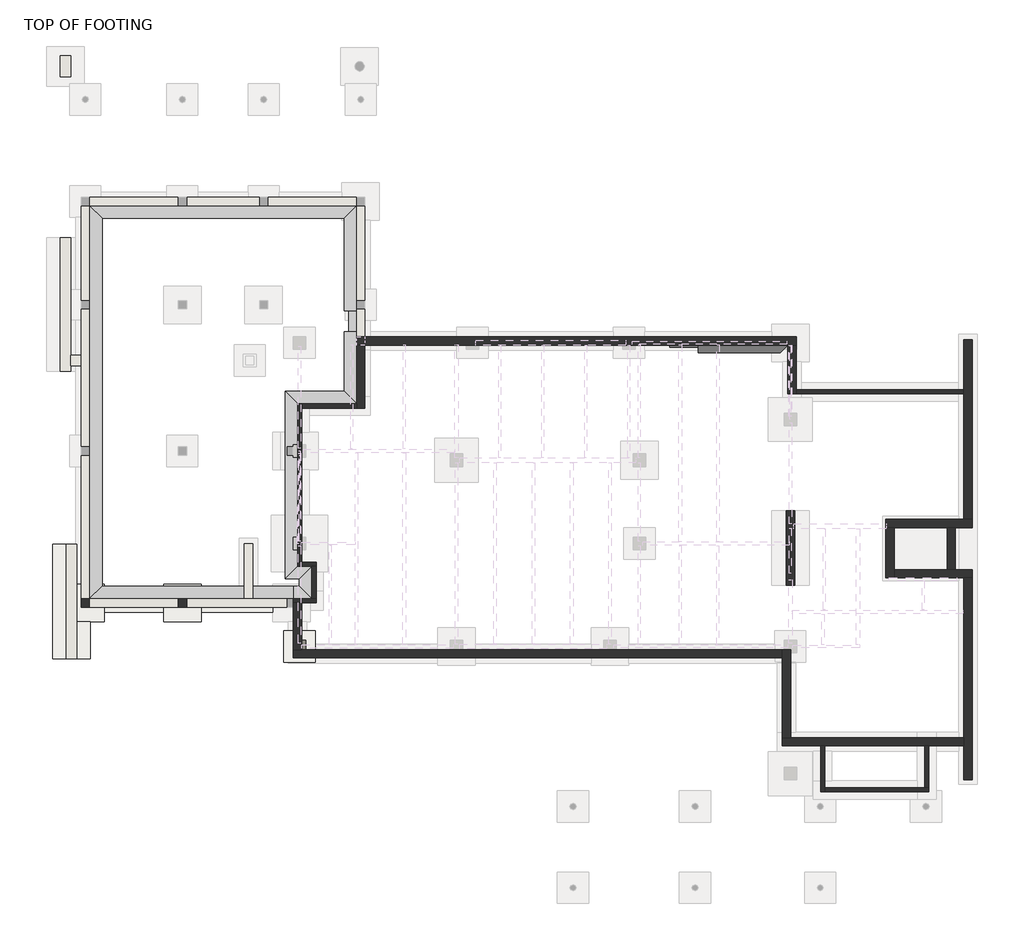
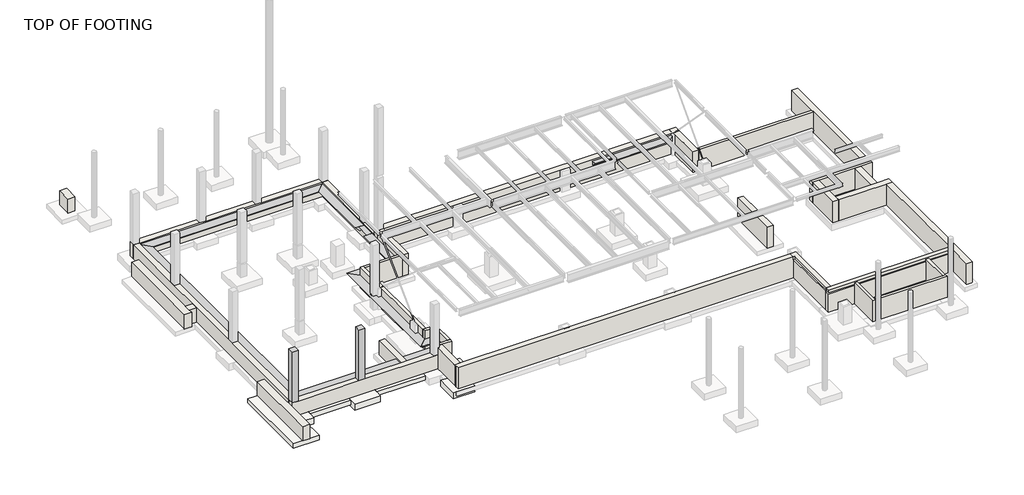
# One storey, part 1 of 4: 32 walls, 8 proxies, 3 slabs, 2 columns, 2 footings.
"""IFC4 building model written with IfcOpenShell, lengths in millimetres."""

from ifc_helpers import new_model, si_unit, frame, origin, place, context, project, spatial, polyline, outline, extrude, faceted_brep, element, save

model = new_model("IFC4")

# Units and contexts
model_context = context("Model", 3, world=origin())
ifc_project = project(units=[si_unit("LENGTHUNIT", "METRE", prefix="MILLI")], contexts=[model_context])

# Site, building, storey
site = spatial("IfcSite", under=ifc_project)
building = spatial("IfcBuilding", under=site)
storey = spatial("IfcBuildingStorey", under=building, Name="TOP OF FOOTING", Elevation=28905.2)

# Proxies
placement = place(None, origin())
element("IfcBuildingElementProxy", 1, Name="Thickened 24\" x 12\"", ObjectType="Thickened 24\" x 12\"", at=placement, inside=storey, context=model_context, shape_type="Brep", body=[
    faceted_brep([(-20560.3454607, 14520.2695005, 29565.6), (-20560.3454607, 14520.2695005, 29870.4), (-19950.7454607, 13910.6695005, 29870.4), (-20255.5454607, 14215.4695005, 29565.6), (-20560.3454607, -4618.6304995, 29565.6), (-20255.5454607, -4313.8304995, 29565.6), (-19950.7454607, -4009.0304995, 29870.4), (-20560.3454607, -4618.6304995, 29870.4)], [[[0, 1, 2, 3]], [[4, 5, 6, 7]], [[1, 0, 4, 7]], [[2, 1, 7, 6]], [[3, 2, 6, 5]], [[0, 3, 5, 4]]]),
])
element("IfcBuildingElementProxy", 2, Name="Thickened 24\" x 12\"", ObjectType="Thickened 24\" x 12\"", at=placement, inside=storey, context=model_context, shape_type="Brep", body=[
    faceted_brep([(-7555.5454607, 9402.1695005, 29565.6), (-7555.5454607, 9402.1695005, 29870.4), (-7923.8454607, 9402.1695005, 29870.4), (-8165.1454607, 9402.1695005, 29870.4), (-7860.3454607, 9402.1695005, 29565.6), (-7619.0454607, 9402.1695005, 29565.6), (-7555.5454607, 14520.2695005, 29565.6), (-7860.3454607, 14215.4695005, 29565.6), (-8165.1454607, 13910.6695005, 29870.4), (-7555.5454607, 14520.2695005, 29870.4)], [[[0, 1, 2, 3, 4, 5]], [[6, 7, 8, 9]], [[1, 0, 6, 9]], [[3, 2, 1, 9, 8]], [[4, 3, 8, 7]], [[0, 5, 4, 7, 6]]]),
])
element("IfcBuildingElementProxy", 3, Name="Thickened 24\" x 12\"", ObjectType="Thickened 24\" x 12\"", at=placement, inside=storey, context=model_context, shape_type="Brep", body=[
    faceted_brep([(-20560.3454607, -4618.6304995, 29565.6), (-20560.3454607, -4618.6304995, 29870.4), (-19950.7454607, -4009.0304995, 29870.4), (-20255.5454607, -4313.8304995, 29565.6), (-10632.1204607, -4618.6304995, 29565.6), (-10632.1204607, -4313.8304995, 29565.6), (-10632.1204607, -4009.0304995, 29870.4), (-10632.1204607, -4618.6304995, 29870.4)], [[[0, 1, 2, 3]], [[4, 5, 6, 7]], [[1, 0, 4, 7]], [[2, 1, 7, 6]], [[3, 2, 6, 5]], [[0, 3, 5, 4]]]),
])
element("IfcBuildingElementProxy", 4, Name="Thickened 24\" x 12\"", ObjectType="Thickened 24\" x 12\"", at=placement, inside=storey, context=model_context, shape_type="Brep", body=[
    faceted_brep([(-10428.9204607, -3040.6554995, 29565.6), (-10428.9204607, -3040.6554995, 29870.4), (-11038.5204607, -3650.2554995, 29870.4), (-10733.7204607, -3345.4554995, 29565.6), (-10428.9204607, 4865.0945005, 29565.6), (-10428.9204607, 4865.0945005, 29870.4), (-11038.5204607, 5474.6945005, 29870.4), (-10733.7204607, 5169.8945005, 29565.6), (-7555.5454607, 4865.0945005, 29565.6), (-7860.3454607, 5169.8945005, 29565.6), (-8165.1454607, 5474.6945005, 29870.4), (-7555.5454607, 4865.0945005, 29870.4)], [[[0, 1, 2, 3]], [[1, 0, 4, 5]], [[2, 1, 5, 6]], [[3, 2, 6, 7]], [[0, 3, 7, 4]], [[8, 9, 10, 11]], [[5, 4, 8, 11]], [[6, 5, 11, 10]], [[7, 6, 10, 9]], [[4, 7, 9, 8]]]),
])
element("IfcBuildingElementProxy", 5, Name="Thickened 24\" x 12\"", ObjectType="Thickened 24\" x 12\"", at=placement, inside=storey, context=model_context, shape_type="Brep", body=[
    faceted_brep([(13450.2545393, 7725.7695005, 30048.2), (13450.2545393, 7725.7695005, 30353.0), (12840.6545393, 7116.1695005, 30353.0), (13145.4545393, 7420.9695005, 30048.2), (9071.9295393, 7725.7695005, 30353.0), (9071.9295393, 7725.7695005, 30048.2), (9071.9295393, 7420.9695005, 30048.2), (9071.9295393, 7116.1695005, 30353.0)], [[[0, 1, 2, 3]], [[4, 5, 6, 7]], [[1, 0, 5, 4]], [[2, 1, 4, 7]], [[3, 2, 7, 6]], [[0, 3, 6, 5]]]),
    faceted_brep([(9071.9295393, 7992.4695005, 30048.2), (9071.9295393, 7992.4695005, 30353.0), (9071.9295393, 7725.7695005, 30353.0), (9071.9295393, 7382.8695005, 30353.0), (9071.9295393, 7687.6695005, 30048.2), (7700.3295393, 7992.4695005, 30353.0), (7700.3295393, 7992.4695005, 30048.2), (7700.3295393, 7725.7695005, 30048.2), (7700.3295393, 7687.6695005, 30048.2), (7700.3295393, 7382.8695005, 30353.0), (7700.3295393, 7725.7695005, 30353.0)], [[[0, 1, 2, 3, 4]], [[5, 6, 7, 8, 9, 10]], [[1, 0, 6, 5]], [[3, 2, 1, 5, 10, 9]], [[4, 3, 9, 8]], [[0, 4, 8, 7, 6]]]),
    faceted_brep([(-7555.5454607, 4865.0945005, 29565.6), (-7555.5454607, 4865.0945005, 29870.4), (-8165.1454607, 5474.6945005, 29870.4), (-7860.3454607, 5169.8945005, 29565.6), (-7555.5454607, 8386.1695005, 29870.4), (-7555.5454607, 8386.1695005, 29565.6), (-7860.3454607, 8386.1695005, 29565.6), (-8165.1454607, 8386.1695005, 29870.4)], [[[0, 1, 2, 3]], [[4, 5, 6, 7]], [[1, 0, 5, 4]], [[2, 1, 4, 7]], [[3, 2, 7, 6]], [[0, 3, 6, 5]]]),
    faceted_brep([(-7314.2454607, 8386.1695005, 29565.6), (-7314.2454607, 8386.1695005, 29870.4), (-7555.5454607, 8386.1695005, 29870.4), (-7923.8454607, 8386.1695005, 29870.4), (-7619.0454607, 8386.1695005, 29565.6), (-7314.2454607, 9402.1695005, 29870.4), (-7314.2454607, 9402.1695005, 29565.6), (-7555.5454607, 9402.1695005, 29565.6), (-7619.0454607, 9402.1695005, 29565.6), (-7923.8454607, 9402.1695005, 29870.4), (-7555.5454607, 9402.1695005, 29870.4)], [[[0, 1, 2, 3, 4]], [[5, 6, 7, 8, 9, 10]], [[1, 0, 6, 5]], [[1, 5, 10, 9, 3, 2]], [[4, 3, 9, 8]], [[0, 4, 8, 7, 6]]]),
    faceted_brep([(-7555.5454607, 14520.2695005, 29565.6), (-7555.5454607, 14520.2695005, 29870.4), (-8165.1454607, 13910.6695005, 29870.4), (-7860.3454607, 14215.4695005, 29565.6), (-20560.3454607, 14520.2695005, 29870.4), (-20560.3454607, 14520.2695005, 29565.6), (-20255.5454607, 14215.4695005, 29565.6), (-19950.7454607, 13910.6695005, 29870.4)], [[[0, 1, 2, 3]], [[4, 5, 6, 7]], [[1, 0, 5, 4]], [[2, 1, 4, 7]], [[3, 2, 7, 6]], [[0, 3, 6, 5]]]),
])
element("IfcBuildingElementProxy", 6, Name="Thickened 24\" x 12\"", ObjectType="Thickened 24\" x 12\"", at=placement, inside=storey, context=model_context, shape_type="Brep", body=[
    faceted_brep([(-10632.1204607, -4618.6304995, 29565.6), (-10632.1204607, -4618.6304995, 29870.4), (-10632.1204607, -4009.0304995, 29870.4), (-10632.1204607, -4313.8304995, 29565.6), (-9727.2454607, -4618.6304995, 29565.6), (-10032.0454607, -4313.8304995, 29565.6), (-10336.8454607, -4009.0304995, 29870.4), (-9727.2454607, -4618.6304995, 29870.4)], [[[0, 1, 2, 3]], [[4, 5, 6, 7]], [[1, 0, 4, 7]], [[2, 1, 7, 6]], [[3, 2, 6, 5]], [[0, 3, 5, 4]]]),
])
element("IfcBuildingElementProxy", 7, Name="Thickened 24\" x 12\"", ObjectType="Thickened 24\" x 12\"", at=placement, inside=storey, context=model_context, shape_type="Brep", body=[
    faceted_brep([(-9727.2454607, -4618.6304995, 29565.6), (-9727.2454607, -4618.6304995, 29870.4), (-10336.8454607, -4009.0304995, 29870.4), (-10032.0454607, -4313.8304995, 29565.6), (-9727.2454607, -3040.6554995, 29565.6), (-10032.0454607, -3345.4554995, 29565.6), (-10336.8454607, -3650.2554995, 29870.4), (-9727.2454607, -3040.6554995, 29870.4)], [[[0, 1, 2, 3]], [[4, 5, 6, 7]], [[1, 0, 4, 7]], [[2, 1, 7, 6]], [[3, 2, 6, 5]], [[0, 3, 5, 4]]]),
])
element("IfcBuildingElementProxy", 8, Name="Thickened 24\" x 12\"", ObjectType="Thickened 24\" x 12\"", at=placement, inside=storey, context=model_context, shape_type="Brep", body=[
    faceted_brep([(-9727.2454607, -3040.6554995, 29565.6), (-9727.2454607, -3040.6554995, 29870.4), (-10336.8454607, -3650.2554995, 29870.4), (-10032.0454607, -3345.4554995, 29565.6), (-10428.9204607, -3040.6554995, 29565.6), (-10733.7204607, -3345.4554995, 29565.6), (-11038.5204607, -3650.2554995, 29870.4), (-10428.9204607, -3040.6554995, 29870.4)], [[[0, 1, 2, 3]], [[4, 5, 6, 7]], [[1, 0, 4, 7]], [[2, 1, 7, 6]], [[3, 2, 6, 5]], [[0, 3, 5, 4]]]),
])

# Columns
element("IfcColumn", 9, ObjectType="Concrete-Rectangular-Column : 16 x 16", at=placement, inside=storey, context=model_context, shape_type="Brep", body=[
    faceted_brep([(-20560.3454607, -4618.6304995, 33782.0), (-20560.3454607, -5025.0304995, 33782.0), (-20560.3454607, -5025.0304995, 29972.0), (-20560.3454607, -4618.6304995, 29972.0), (-20966.7454607, -5025.0304995, 33782.0), (-20966.7454607, -5025.0304995, 29972.0), (-20966.7454607, -4720.2304995, 33782.0), (-20966.7454607, -4618.6304995, 33782.0), (-20966.7454607, -4618.6304995, 29972.0)], [[[0, 1, 2, 3]], [[1, 4, 5, 2]], [[4, 6, 7, 8, 5]], [[7, 0, 3, 8]], [[1, 0, 7, 6, 4]], [[3, 2, 5, 8]]]),
])
element("IfcColumn", 10, ObjectType="Concrete-Rectangular-Column : 16 x 16", at=placement, inside=storey, context=model_context, shape_type="SweptSolid", body=[
    extrude(outline(polyline([(-15835.9454607, -4618.6304995), (-15835.9454607, -5025.0304995), (-16242.3454607, -5025.0304995), (-16242.3454607, -4618.6304995), (-15835.9454607, -4618.6304995)])), frame((0.0, 0.0, 29972.0), z_axis=(0.0, 0.0, 1.0), x_axis=(1.0, 0.0, 0.0)), (0.0, 0.0, 1.0), 3810.0),
])

# Footings
element("IfcFooting", 11, ObjectType="Bearing Footing - 36\" x 12\"", at=placement, inside=storey, context=model_context, shape_type="Brep", body=[
    faceted_brep([(-19849.1454607, -4364.6304995, 28905.2), (-19849.1454607, -5279.0304995, 28905.2), (-16953.5454607, -5279.0304995, 28905.2), (-16953.5454607, -4364.6304995, 28905.2), (-19849.1454607, -5279.0304995, 28600.4), (-16953.5454607, -5279.0304995, 28600.4), (-19849.1454607, -4364.6304995, 28600.4), (-16953.5454607, -4364.6304995, 28600.4)], [[[0, 1, 2, 3]], [[1, 4, 5, 2]], [[4, 6, 7, 5]], [[6, 0, 3, 7]], [[1, 0, 6, 4]], [[3, 2, 5, 7]]]),
    faceted_brep([(-15124.7454607, -4364.6304995, 28905.2), (-15124.7454607, -5279.0304995, 28905.2), (-11647.3763201, -5279.0304995, 28905.2), (-11647.3763201, -4364.6304995, 28905.2), (-12354.5579607, -4364.6304995, 28905.2), (-13268.9579607, -4364.6304995, 28905.2), (-15124.7454607, -5279.0304995, 28600.4), (-11647.3763201, -5279.0304995, 28600.4), (-15124.7454607, -4364.6304995, 28600.4), (-13268.9579607, -4364.6304995, 28600.4), (-12354.5579607, -4364.6304995, 28600.4), (-11647.3763201, -4364.6304995, 28600.4)], [[[0, 1, 2, 3, 4, 5]], [[1, 6, 7, 2]], [[6, 8, 9, 10, 11, 7]], [[8, 0, 5, 4, 3, 11, 10, 9]], [[1, 0, 8, 6]], [[3, 2, 7, 11]]]),
])
element("IfcFooting", 12, ObjectType="Bearing Footing - 72\" x 12\" 2", at=placement, inside=storey, context=model_context, shape_type="SweptSolid", body=[
    extrude(outline(polyline([(-20517.4622482, -7552.3304995), (-22346.2622482, -7552.3304995), (-22346.2622482, -1964.3304995), (-21220.7454607, -1964.3304995), (-21220.7454607, -3907.4304995), (-21677.9454607, -3907.4304995), (-21677.9454607, -5736.2304995), (-20517.4622482, -5736.2304995), (-20517.4622482, -7552.3304995)])), frame((0.0, 0.0, 28600.4), z_axis=(0.0, 0.0, 1.0), x_axis=(1.0, 0.0, 0.0)), (0.0, 0.0, 1.0), 304.8),
])

# Slabs
element("IfcSlab", 13, ObjectType="Footing-Rectangular : 6'-0\" x 6'-0\" x 1'-6\"", at=placement, inside=storey, context=model_context, shape_type="Brep", body=[
    faceted_brep([(-19849.1454607, -3907.4304995, 28905.2), (-20306.3454607, -3907.4304995, 28905.2), (-21220.7454607, -3907.4304995, 28905.2), (-21677.9454607, -3907.4304995, 28905.2), (-21677.9454607, -5736.2304995, 28905.2), (-20517.4622482, -5736.2304995, 28905.2), (-19849.1454607, -5736.2304995, 28905.2), (-19849.1454607, -5279.0304995, 28905.2), (-19849.1454607, -4364.6304995, 28905.2), (-19849.1454607, -3907.4304995, 28448.0), (-19849.1454607, -5736.2304995, 28448.0), (-21677.9454607, -5736.2304995, 28448.0), (-21677.9454607, -3907.4304995, 28448.0), (-21677.9454607, -3907.4304995, 28600.4), (-21677.9454607, -5736.2304995, 28600.4)], [[[0, 1, 2, 3, 4, 5, 6, 7, 8]], [[9, 10, 11, 12]], [[3, 2, 1, 0, 9, 12, 13]], [[4, 3, 13, 12, 11, 14]], [[6, 5, 4, 14, 11, 10]], [[0, 8, 7, 6, 10, 9]]]),
])
element("IfcSlab", 14, ObjectType="Footing-Rectangular : 6'-0\" x 6'-0\" x 1'-6\"", at=placement, inside=storey, context=model_context, shape_type="Brep", body=[
    faceted_brep([(-15124.7454607, -3907.4304995, 28905.2), (-16953.5454607, -3907.4304995, 28905.2), (-16953.5454607, -4364.6304995, 28905.2), (-16953.5454607, -5279.0304995, 28905.2), (-16953.5454607, -5736.2304995, 28905.2), (-15124.7454607, -5736.2304995, 28905.2), (-15124.7454607, -5279.0304995, 28905.2), (-15124.7454607, -4364.6304995, 28905.2), (-15124.7454607, -3907.4304995, 28448.0), (-15124.7454607, -5736.2304995, 28448.0), (-16953.5454607, -5736.2304995, 28448.0), (-16953.5454607, -3907.4304995, 28448.0)], [[[0, 1, 2, 3, 4, 5, 6, 7]], [[8, 9, 10, 11]], [[1, 0, 8, 11]], [[4, 3, 2, 1, 11, 10]], [[5, 4, 10, 9]], [[0, 7, 6, 5, 9, 8]]]),
])
element("IfcSlab", 15, ObjectType="Footing-Rectangular_With_Pier : F1 - 5'-0\" x 5'-0\" x 1'-6\"", at=placement, inside=storey, context=model_context, shape_type="SolidModel", body=[
    extrude(outline(polyline([(-10022.5204607, -6637.9304995), (-10022.5204607, -7247.5304995), (-10632.1204607, -7247.5304995), (-10632.1204607, -6637.9304995), (-10022.5204607, -6637.9304995)])), frame((0.0, 0.0, 28905.2), z_axis=(0.0, 0.0, 1.0), x_axis=(1.0, 0.0, 0.0)), (0.0, 0.0, 1.0), 1549.4),
    faceted_brep([(-9565.3204607, -6180.7304995, 28905.2), (-9971.7204607, -6180.7304995, 28905.2), (-10886.1204607, -6180.7304995, 28905.2), (-11089.3204607, -6180.7304995, 28905.2), (-11089.3204607, -7704.7304995, 28905.2), (-10886.1204607, -7704.7304995, 28905.2), (-9565.3204607, -7704.7304995, 28905.2), (-9565.3204607, -6841.1304995, 28905.2), (-9565.3204607, -6180.7304995, 28448.0), (-9565.3204607, -7704.7304995, 28448.0), (-11089.3204607, -7704.7304995, 28448.0), (-11089.3204607, -6180.7304995, 28448.0), (-9565.3204607, -7704.7304995, 28600.4)], [[[0, 1, 2, 3, 4, 5, 6, 7]], [[8, 9, 10, 11]], [[3, 2, 1, 0, 8, 11]], [[4, 3, 11, 10]], [[6, 5, 4, 10, 9, 12]], [[0, 7, 6, 12, 9, 8]]]),
])

# Walls
element("IfcWall", 16, ObjectType="Foundation - 16\" Concrete", at=placement, inside=storey, context=model_context, shape_type="Brep", body=[
    faceted_brep([(-7555.5454607, 7725.7695005, 28905.2), (-7149.1454607, 7725.7695005, 28905.2), (13450.2545393, 7725.7695005, 28905.2), (13856.6545393, 7725.7695005, 28905.2), (13856.6545393, 7725.7695005, 30480.0), (13450.2545393, 7725.7695005, 30480.0), (-7149.1454607, 7725.7695005, 30480.0), (-7555.5454607, 7725.7695005, 30480.0), (-7555.5454607, 8132.1695005, 28905.2), (-7555.5454607, 8132.1695005, 29972.0), (-7555.5454607, 8132.1695005, 30480.0), (-7149.1454607, 8132.1695005, 30480.0), (13856.6545393, 8132.1695005, 30480.0), (13856.6545393, 8132.1695005, 28905.2), (-7149.1454607, 8132.1695005, 28905.2)], [[[0, 1, 2, 3, 4, 5, 6, 7]], [[8, 9, 10, 11, 12, 13, 14]], [[3, 2, 1, 0, 8, 14, 13]], [[7, 6, 5, 4, 12, 11, 10]], [[4, 3, 13, 12]], [[0, 7, 10, 9, 8]]]),
])
element("IfcWall", 17, ObjectType="Foundation - 16\" Concrete", at=placement, inside=storey, context=model_context, shape_type="Brep", body=[
    faceted_brep([(13450.2545393, 7725.7695005, 28905.2), (13450.2545393, 5350.8695005, 28905.2), (13450.2545393, 5350.8695005, 30480.0), (13450.2545393, 7725.7695005, 30480.0), (13856.6545393, 7725.7695005, 28905.2), (13856.6545393, 7725.7695005, 30480.0), (13856.6545393, 5554.0695005, 30480.0), (13856.6545393, 5350.8695005, 30480.0), (13856.6545393, 5350.8695005, 28905.2), (13856.6545393, 5554.0695005, 28905.2)], [[[0, 1, 2, 3]], [[4, 5, 6, 7, 8, 9]], [[1, 0, 4, 9, 8]], [[3, 2, 7, 6, 5]], [[0, 3, 5, 4]], [[2, 1, 8, 7]]]),
])
element("IfcWall", 18, ObjectType="Foundation - 16\" Concrete", at=placement, inside=storey, context=model_context, shape_type="Brep", body=[
    faceted_brep([(22019.578935, 7995.5948911, 28905.2), (22019.578935, 5554.0695005, 28905.2), (22019.578935, 5350.8695005, 28905.2), (22019.578935, -757.8304995, 28905.2), (22019.578935, -757.8304995, 30480.0), (22019.578935, 5350.8695005, 30480.0), (22019.578935, 5554.0695005, 30480.0), (22019.578935, 7995.5948911, 30480.0), (22425.978935, 7995.5948911, 28905.2), (22425.978935, 7995.5948911, 30480.0), (22425.978935, -757.8304995, 30480.0), (22425.978935, -757.8304995, 28905.2)], [[[0, 1, 2, 3, 4, 5, 6, 7]], [[8, 9, 10, 11]], [[3, 2, 1, 0, 8, 11]], [[7, 6, 5, 4, 10, 9]], [[0, 7, 9, 8]], [[4, 3, 11, 10]]]),
])
element("IfcWall", 19, ObjectType="Foundation - 16\" Concrete", at=placement, inside=storey, context=model_context, shape_type="Brep", body=[
    faceted_brep([(13177.2045393, -7095.1304995, 28905.2), (-10225.7204607, -7095.1304995, 28905.2), (-10632.1204607, -7095.1304995, 28905.2), (-10632.1204607, -7095.1304995, 30480.0), (-10225.7204607, -7095.1304995, 30480.0), (13177.2045393, -7095.1304995, 30480.0), (13177.2045393, -7501.5304995, 28905.2), (13177.2045393, -7501.5304995, 30276.8), (13177.2045393, -7501.5304995, 30480.0), (-10632.1204607, -7501.5304995, 30480.0), (-10632.1204607, -7501.5304995, 28905.2)], [[[0, 1, 2, 3, 4, 5]], [[6, 7, 8, 9, 10]], [[2, 1, 0, 6, 10]], [[5, 4, 3, 9, 8]], [[3, 2, 10, 9]], [[0, 5, 8, 7, 6]]]),
])
element("IfcWall", 20, ObjectType="Foundation - 16\" Concrete", at=placement, inside=storey, context=model_context, shape_type="Brep", body=[
    faceted_brep([(-10225.7204607, -7095.1304995, 28905.2), (-10225.7204607, -4821.8304995, 28905.2), (-10225.7204607, -4821.8304995, 30480.0), (-10225.7204607, -7095.1304995, 30480.0), (-10632.1204607, -7095.1304995, 28905.2), (-10632.1204607, -7095.1304995, 30480.0), (-10632.1204607, -5025.0304995, 30480.0), (-10632.1204607, -4821.8304995, 30480.0), (-10632.1204607, -4821.8304995, 28905.2)], [[[0, 1, 2, 3]], [[4, 5, 6, 7, 8]], [[1, 0, 4, 8]], [[3, 2, 7, 6, 5]], [[0, 3, 5, 4]], [[2, 1, 8, 7]]]),
])
element("IfcWall", 21, ObjectType="Foundation - 16\" Concrete", at=placement, inside=storey, context=model_context, shape_type="Brep", body=[
    faceted_brep([(22425.978935, -757.8304995, 28905.2), (22019.578935, -757.8304995, 28905.2), (18219.8486799, -757.8304995, 28905.2), (18219.8486799, -757.8304995, 30480.0), (22019.578935, -757.8304995, 30480.0), (22425.978935, -757.8304995, 30480.0), (22425.978935, -1164.2304995, 28905.2), (22425.978935, -1164.2304995, 30480.0), (21605.9861799, -1164.2304995, 30480.0), (21199.5861799, -1164.2304995, 30480.0), (18626.2486799, -1164.2304995, 30480.0), (18219.8486799, -1164.2304995, 30480.0), (18219.8486799, -1164.2304995, 28905.2), (18626.2486799, -1164.2304995, 28905.2), (21199.5861799, -1164.2304995, 28905.2), (21605.9861799, -1164.2304995, 28905.2)], [[[0, 1, 2, 3, 4, 5]], [[6, 7, 8, 9, 10, 11, 12, 13, 14, 15]], [[2, 1, 0, 6, 15, 14, 13, 12]], [[5, 4, 3, 11, 10, 9, 8, 7]], [[0, 5, 7, 6]], [[3, 2, 12, 11]]]),
])
element("IfcWall", 22, ObjectType="Foundation - 16\" Concrete", at=placement, inside=storey, context=model_context, shape_type="Brep", body=[
    faceted_brep([(-20966.7454607, 14520.2695005, 28905.2), (-20560.3454607, 14520.2695005, 28905.2), (-7555.5454607, 14520.2695005, 28905.2), (-7149.1454607, 14520.2695005, 28905.2), (-7149.1454607, 14520.2695005, 29972.0), (-7555.5454607, 14520.2695005, 29972.0), (-11873.5454607, 14520.2695005, 29972.0), (-12279.9454607, 14520.2695005, 29972.0), (-15835.9454607, 14520.2695005, 29972.0), (-16242.3454607, 14520.2695005, 29972.0), (-20560.3454607, 14520.2695005, 29972.0), (-20966.7454607, 14520.2695005, 29972.0), (-20966.7454607, 14926.6695005, 28905.2), (-20966.7454607, 14926.6695005, 29972.0), (-20560.3454607, 14926.6695005, 29972.0), (-16242.3454607, 14926.6695005, 29972.0), (-15835.9454607, 14926.6695005, 29972.0), (-12279.9454607, 14926.6695005, 29972.0), (-11873.5454607, 14926.6695005, 29972.0), (-7555.5454607, 14926.6695005, 29972.0), (-7149.1454607, 14926.6695005, 29972.0), (-7149.1454607, 14926.6695005, 28905.2)], [[[0, 1, 2, 3, 4, 5, 6, 7, 8, 9, 10, 11]], [[12, 13, 14, 15, 16, 17, 18, 19, 20, 21]], [[3, 2, 1, 0, 12, 21]], [[11, 10, 9, 8, 7, 6, 5, 4, 20, 19, 18, 17, 16, 15, 14, 13]], [[4, 3, 21, 20]], [[0, 11, 13, 12]]]),
])
element("IfcWall", 23, ObjectType="Foundation - 16\" Concrete", at=placement, inside=storey, context=model_context, shape_type="Brep", body=[
    faceted_brep([(-7555.5454607, 14520.2695005, 28905.2), (-7555.5454607, 8132.1695005, 28905.2), (-7555.5454607, 8132.1695005, 29972.0), (-7555.5454607, 9491.0695005, 29972.0), (-7555.5454607, 9897.4695005, 29972.0), (-7555.5454607, 14520.2695005, 29972.0), (-7149.1454607, 14520.2695005, 28905.2), (-7149.1454607, 14520.2695005, 29972.0), (-7149.1454607, 9897.4695005, 29972.0), (-7149.1454607, 9491.0695005, 29972.0), (-7149.1454607, 8132.1695005, 29972.0), (-7149.1454607, 8132.1695005, 28905.2)], [[[0, 1, 2, 3, 4, 5]], [[6, 7, 8, 9, 10, 11]], [[1, 0, 6, 11]], [[5, 4, 3, 2, 10, 9, 8, 7]], [[0, 5, 7, 6]], [[2, 1, 11, 10]]]),
])
element("IfcWall", 24, ObjectType="Foundation - 16\" Concrete", at=placement, inside=storey, context=model_context, shape_type="Brep", body=[
    faceted_brep([(-10632.1204607, -4618.6304995, 28905.2), (-12608.5579607, -4618.6304995, 28905.2), (-13014.9579607, -4618.6304995, 28905.2), (-20560.3454607, -4618.6304995, 28905.2), (-20966.7454607, -4618.6304995, 28905.2), (-20966.7454607, -4618.6304995, 29972.0), (-20560.3454607, -4618.6304995, 29972.0), (-16242.3454607, -4618.6304995, 29972.0), (-15835.9454607, -4618.6304995, 29972.0), (-13014.9579607, -4618.6304995, 29972.0), (-12608.5579607, -4618.6304995, 29972.0), (-10936.1763201, -4618.6304995, 29972.0), (-10632.1204607, -4618.6304995, 29972.0), (-10632.1204607, -5025.0304995, 28905.2), (-10632.1204607, -5025.0304995, 29972.0), (-10936.1763201, -5025.0304995, 29972.0), (-15835.9454607, -5025.0304995, 29972.0), (-16242.3454607, -5025.0304995, 29972.0), (-20560.3454607, -5025.0304995, 29972.0), (-20966.7454607, -5025.0304995, 29972.0), (-20966.7454607, -5025.0304995, 28905.2)], [[[0, 1, 2, 3, 4, 5, 6, 7, 8, 9, 10, 11, 12]], [[13, 14, 15, 16, 17, 18, 19, 20]], [[4, 3, 2, 1, 0, 13, 20]], [[12, 11, 10, 9, 8, 7, 6, 5, 19, 18, 17, 16, 15, 14]], [[0, 12, 14, 13]], [[5, 4, 20, 19]]]),
])
element("IfcWall", 25, ObjectType="Foundation - 16\" Concrete", at=placement, inside=storey, context=model_context, shape_type="Brep", body=[
    faceted_brep([(-20560.3454607, -4618.6304995, 28905.2), (-20560.3454607, 14520.2695005, 28905.2), (-20560.3454607, 14520.2695005, 29972.0), (-20560.3454607, 9897.4695005, 29972.0), (-20560.3454607, 9491.0695005, 29972.0), (-20560.3454607, 2785.4695005, 29972.0), (-20560.3454607, 2379.0695005, 29972.0), (-20560.3454607, -4618.6304995, 29972.0), (-20966.7454607, -4618.6304995, 28905.2), (-20966.7454607, -4618.6304995, 29972.0), (-20966.7454607, 2379.0695005, 29972.0), (-20966.7454607, 2785.4695005, 29972.0), (-20966.7454607, 6722.4695005, 29972.0), (-20966.7454607, 7230.4695005, 29972.0), (-20966.7454607, 9491.0695005, 29972.0), (-20966.7454607, 9897.4695005, 29972.0), (-20966.7454607, 14520.2695005, 29972.0), (-20966.7454607, 14520.2695005, 28905.2), (-20966.7454607, 7230.4695005, 28905.2), (-20966.7454607, 6722.4695005, 28905.2)], [[[0, 1, 2, 3, 4, 5, 6, 7]], [[8, 9, 10, 11, 12, 13, 14, 15, 16, 17, 18, 19]], [[1, 0, 8, 19, 18, 17]], [[7, 6, 5, 4, 3, 2, 16, 15, 14, 13, 12, 11, 10, 9]], [[0, 7, 9, 8]], [[2, 1, 17, 16]]]),
])
element("IfcWall", 26, ObjectType="Foundation - 16\" Concrete", at=placement, inside=storey, context=model_context, shape_type="Brep", body=[
    faceted_brep([(-7555.5454607, 7725.7695005, 30480.0), (-7555.5454607, 7725.7695005, 28905.2), (-7555.5454607, 4865.0945005, 28905.2), (-7555.5454607, 4661.8945005, 28905.2), (-7555.5454607, 4661.8945005, 30480.0), (-7555.5454607, 4865.0945005, 30480.0), (-7149.1454607, 7725.7695005, 28905.2), (-7149.1454607, 7725.7695005, 30480.0), (-7149.1454607, 4661.8945005, 30480.0), (-7149.1454607, 4661.8945005, 28905.2)], [[[0, 1, 2, 3, 4, 5]], [[6, 7, 8, 9]], [[3, 2, 1, 6, 9]], [[0, 5, 4, 8, 7]], [[4, 3, 9, 8]], [[0, 7, 6, 1]]]),
])
element("IfcWall", 27, ObjectType="Foundation - 16\" Concrete", at=placement, inside=storey, context=model_context, shape_type="Brep", body=[
    faceted_brep([(18626.2486799, -3602.6304995, 28905.2), (18626.2486799, -3196.2304995, 28905.2), (18626.2486799, -1164.2304995, 28905.2), (18626.2486799, -1164.2304995, 30480.0), (18626.2486799, -3196.2304995, 30480.0), (18626.2486799, -3602.6304995, 30480.0), (18219.8486799, -3602.6304995, 28905.2), (18219.8486799, -3602.6304995, 30480.0), (18219.8486799, -1164.2304995, 30480.0), (18219.8486799, -1164.2304995, 28905.2)], [[[0, 1, 2, 3, 4, 5]], [[6, 7, 8, 9]], [[2, 1, 0, 6, 9]], [[5, 4, 3, 8, 7]], [[0, 5, 7, 6]], [[3, 2, 9, 8]]]),
])
element("IfcWall", 28, ObjectType="Foundation - 16\" Concrete", at=placement, inside=storey, context=model_context, shape_type="Brep", body=[
    faceted_brep([(18626.2486799, -3602.6304995, 28905.2), (22019.578935, -3602.6304995, 28905.2), (22425.978935, -3602.6304995, 28905.2), (22425.978935, -3602.6304995, 30480.0), (22019.578935, -3602.6304995, 30480.0), (18626.2486799, -3602.6304995, 30480.0), (18626.2486799, -3196.2304995, 28905.2), (18626.2486799, -3196.2304995, 30480.0), (21199.5861799, -3196.2304995, 30480.0), (21605.9861799, -3196.2304995, 30480.0), (22425.978935, -3196.2304995, 30480.0), (22425.978935, -3196.2304995, 28905.2), (21605.9861799, -3196.2304995, 28905.2), (21199.5861799, -3196.2304995, 28905.2)], [[[0, 1, 2, 3, 4, 5]], [[6, 7, 8, 9, 10, 11, 12, 13]], [[2, 1, 0, 6, 13, 12, 11]], [[5, 4, 3, 10, 9, 8, 7]], [[0, 5, 7, 6]], [[3, 2, 11, 10]]]),
])
element("IfcWall", 29, ObjectType="Foundation - 16\" Concrete", at=placement, inside=storey, context=model_context, shape_type="SweptSolid", body=[
    extrude(outline(polyline([(21605.9861799, -1164.2304995), (21605.9861799, -3196.2304995), (21199.5861799, -3196.2304995), (21199.5861799, -1164.2304995), (21605.9861799, -1164.2304995)])), frame((0.0, 0.0, 28905.2), z_axis=(0.0, 0.0, 1.0), x_axis=(1.0, 0.0, 0.0)), (0.0, 0.0, 1.0), 1574.8),
])
element("IfcWall", 30, ObjectType="Foundation - 16\" Concrete", at=placement, inside=storey, context=model_context, shape_type="SweptSolid", body=[
    extrude(outline(polyline([(-12608.5579607, -1935.7554995), (-12608.5579607, -4618.6304995), (-13014.9579607, -4618.6304995), (-13014.9579607, -1935.7554995), (-12608.5579607, -1935.7554995)])), frame((0.0, 0.0, 28905.2), z_axis=(0.0, 0.0, 1.0), x_axis=(1.0, 0.0, 0.0)), (0.0, 0.0, 1.0), 1066.8),
])
element("IfcWall", 31, ObjectType="Foundation - 16\" Concrete", at=placement, inside=storey, context=model_context, shape_type="Brep", body=[
    faceted_brep([(22019.578935, -3602.6304995, 28905.2), (22019.578935, -11381.3804995, 28905.2), (22019.578935, -11787.7804995, 28905.2), (22019.578935, -13445.1304995, 28905.2), (22019.578935, -13445.1304995, 30480.0), (22019.578935, -11686.1804995, 30480.0), (22019.578935, -11381.3804995, 30480.0), (22019.578935, -3602.6304995, 30480.0), (22425.978935, -3602.6304995, 28905.2), (22425.978935, -3602.6304995, 30480.0), (22425.978935, -13445.1304995, 30480.0), (22425.978935, -13445.1304995, 28905.2)], [[[0, 1, 2, 3, 4, 5, 6, 7]], [[8, 9, 10, 11]], [[3, 2, 1, 0, 8, 11]], [[4, 3, 11, 10]], [[7, 6, 5, 4, 10, 9]], [[0, 7, 9, 8]]]),
])
element("IfcWall", 32, ObjectType="Foundation - 16\" Concrete", at=placement, inside=storey, context=model_context, shape_type="SweptSolid", body=[
    extrude(outline(polyline([(13364.5295393, -3958.2304995), (13364.5295393, -326.0304995), (13770.9295393, -326.0304995), (13770.9295393, -3958.2304995), (13364.5295393, -3958.2304995)])), frame((0.0, 0.0, 28905.2), z_axis=(0.0, 0.0, 1.0), x_axis=(1.0, 0.0, 0.0)), (0.0, 0.0, 1.0), 1574.8),
])
element("IfcWall", 33, ObjectType="Foundation - 16\" Concrete w/Brick Ledge", at=placement, inside=storey, context=model_context, shape_type="Brep", body=[
    faceted_brep([(22019.578935, -11381.3804995, 28905.2), (13583.6045393, -11381.3804995, 28905.2), (13177.2045393, -11381.3804995, 28905.2), (13177.2045393, -11381.3804995, 30276.8), (13278.8045393, -11381.3804995, 30276.8), (13278.8045393, -11381.3804995, 30480.0), (13583.6045393, -11381.3804995, 30480.0), (22019.578935, -11381.3804995, 30480.0), (13177.2045393, -11787.7804995, 28905.2), (15037.7545393, -11787.7804995, 28905.2), (15240.9545393, -11787.7804995, 28905.2), (20105.0545393, -11787.7804995, 28905.2), (20308.2545393, -11787.7804995, 28905.2), (22019.578935, -11787.7804995, 28905.2), (22019.578935, -11787.7804995, 30276.8), (13177.2045393, -11787.7804995, 30276.8), (13278.8045393, -11686.1804995, 30480.0), (22019.578935, -11686.1804995, 30480.0), (13278.8045393, -11686.1804995, 30276.8), (22019.578935, -11686.1804995, 30276.8)], [[[0, 1, 2, 3, 4, 5, 6, 7]], [[8, 9, 10, 11, 12, 13, 14, 15]], [[2, 1, 0, 13, 12, 11, 10, 9, 8]], [[7, 6, 5, 16, 17]], [[2, 8, 15, 3]], [[18, 19, 17, 16]], [[19, 18, 4, 3, 15, 14]], [[18, 16, 5, 4]], [[0, 7, 17, 19, 14, 13]]]),
])
element("IfcWall", 34, ObjectType="Foundation - 16\" Concrete w/Brick Ledge", at=placement, inside=storey, context=model_context, shape_type="Brep", body=[
    faceted_brep([(13583.6045393, -11381.3804995, 28905.2), (13583.6045393, -7095.1304995, 28905.2), (13583.6045393, -7095.1304995, 30480.0), (13583.6045393, -11381.3804995, 30480.0), (13177.2045393, -7095.1304995, 28905.2), (13177.2045393, -7501.5304995, 28905.2), (13177.2045393, -11381.3804995, 28905.2), (13177.2045393, -11381.3804995, 30276.8), (13177.2045393, -7501.5304995, 30276.8), (13177.2045393, -7501.5304995, 30480.0), (13177.2045393, -7095.1304995, 30480.0), (13278.8045393, -7501.5304995, 30480.0), (13278.8045393, -11381.3804995, 30480.0), (13278.8045393, -11381.3804995, 30276.8), (13278.8045393, -7501.5304995, 30276.8)], [[[0, 1, 2, 3]], [[4, 5, 6, 7, 8, 9, 10]], [[1, 0, 6, 5, 4]], [[3, 2, 10, 9, 11, 12]], [[2, 1, 4, 10]], [[0, 3, 12, 13, 7, 6]], [[8, 14, 11, 9]], [[11, 14, 13, 12]], [[14, 8, 7, 13]]]),
])
element("IfcWall", 35, ObjectType="Foundation - 20\" Concrete", at=placement, inside=storey, context=model_context, shape_type="Brep", body=[
    faceted_brep([(-21990.9734711, 12968.7995005, 28905.2), (-21990.9734711, 6469.2695005, 28905.2), (-21990.9734711, 6469.2695005, 29972.0), (-21990.9734711, 12968.7995005, 29972.0), (-21482.9734711, 12968.7995005, 28905.2), (-21482.9734711, 12968.7995005, 29972.0), (-21482.9734711, 7230.4695005, 29972.0), (-21482.9734711, 6722.4695005, 29972.0), (-21482.9734711, 6469.2695005, 29972.0), (-21482.9734711, 6469.2695005, 28905.2), (-21482.9734711, 6722.4695005, 28905.2), (-21482.9734711, 7230.4695005, 28905.2)], [[[0, 1, 2, 3]], [[4, 5, 6, 7, 8, 9, 10, 11]], [[1, 0, 4, 11, 10, 9]], [[2, 1, 9, 8]], [[3, 2, 8, 7, 6, 5]], [[0, 3, 5, 4]]]),
])
element("IfcWall", 36, ObjectType="Foundation - 20\" Concrete", at=placement, inside=storey, context=model_context, shape_type="SweptSolid", body=[
    extrude(outline(polyline([(-21685.8622482, -7552.3304995), (-21685.8622482, -1964.3304995), (-21177.8622482, -1964.3304995), (-21177.8622482, -7552.3304995), (-21685.8622482, -7552.3304995)])), frame((0.0, 0.0, 28905.2), z_axis=(0.0, 0.0, 1.0), x_axis=(1.0, 0.0, 0.0)), (0.0, 0.0, 1.0), 1066.8),
])
element("IfcWall", 37, ObjectType="Foundation - 20\" Concrete", at=placement, inside=storey, context=model_context, shape_type="SweptSolid", body=[
    extrude(outline(polyline([(-21990.9919313, 20797.4082736), (-21990.9919313, 21813.4082736), (-21482.9919313, 21813.4082736), (-21482.9919313, 20797.4082736), (-21990.9919313, 20797.4082736)])), frame((0.0, 0.0, 28905.2), z_axis=(0.0, 0.0, 1.0), x_axis=(1.0, 0.0, 0.0)), (0.0, 0.0, 1.0), 1066.8),
])
element("IfcWall", 38, ObjectType="Foundation - 20\" Concrete", at=placement, inside=storey, context=model_context, shape_type="SweptSolid", body=[
    extrude(outline(polyline([(-20966.7454607, 6722.4695005), (-21482.9734711, 6722.4695005), (-21482.9734711, 7230.4695005), (-20966.7454607, 7230.4695005), (-20966.7454607, 6722.4695005)])), frame((0.0, 0.0, 28905.2), z_axis=(0.0, 0.0, 1.0), x_axis=(1.0, 0.0, 0.0)), (0.0, 0.0, 1.0), 1066.8),
])
element("IfcWall", 39, ObjectType="Foundation - 8\" Concrete", at=placement, inside=storey, context=model_context, shape_type="SweptSolid", body=[
    extrude(outline(polyline([(22019.578935, 5350.8695005), (13856.6545393, 5350.8695005), (13856.6545393, 5554.0695005), (22019.578935, 5554.0695005), (22019.578935, 5350.8695005)])), frame((0.0, 0.0, 28905.2), z_axis=(0.0, 0.0, 1.0), x_axis=(1.0, 0.0, 0.0)), (0.0, 0.0, 1.0), 1574.8),
])
element("IfcWall", 40, ObjectType="Foundation - 8\" Concrete", at=placement, inside=storey, context=model_context, shape_type="Brep", body=[
    faceted_brep([(-10225.7204607, -2837.4554995, 28905.2), (-10225.7204607, 4661.8945005, 28905.2), (-10225.7204607, 4865.0945005, 28905.2), (-10225.7204607, 4865.0945005, 30480.0), (-10225.7204607, 4661.8945005, 30480.0), (-10225.7204607, -2837.4554995, 30480.0), (-10428.9204607, -2837.4554995, 28905.2), (-10428.9204607, -2837.4554995, 30480.0), (-10428.9204607, 4865.0945005, 30480.0), (-10428.9204607, 4865.0945005, 28905.2)], [[[0, 1, 2, 3, 4, 5]], [[6, 7, 8, 9]], [[2, 1, 0, 6, 9]], [[5, 4, 3, 8, 7]], [[3, 2, 9, 8]], [[0, 5, 7, 6]]]),
])
element("IfcWall", 41, ObjectType="Foundation - 8\" Concrete", at=placement, inside=storey, context=model_context, shape_type="SweptSolid", body=[
    extrude(outline(polyline([(-10225.7204607, 4865.0945005), (-7555.5454607, 4865.0945005), (-7555.5454607, 4661.8945005), (-10225.7204607, 4661.8945005), (-10225.7204607, 4865.0945005)])), frame((0.0, 0.0, 28905.2), z_axis=(0.0, 0.0, 1.0), x_axis=(1.0, 0.0, 0.0)), (0.0, 0.0, 1.0), 1574.8),
])
element("IfcWall", 42, ObjectType="Foundation - 8\" Concrete", at=placement, inside=storey, context=model_context, shape_type="Brep", body=[
    faceted_brep([(-10428.9204607, -3040.6554995, 28905.2), (-9727.2454607, -3040.6554995, 28905.2), (-9524.0454607, -3040.6554995, 28905.2), (-9524.0454607, -3040.6554995, 30480.0), (-9727.2454607, -3040.6554995, 30480.0), (-10428.9204607, -3040.6554995, 30480.0), (-10428.9204607, -2837.4554995, 28905.2), (-10428.9204607, -2837.4554995, 30480.0), (-10225.7204607, -2837.4554995, 30480.0), (-9524.0454607, -2837.4554995, 30480.0), (-9524.0454607, -2837.4554995, 28905.2), (-10225.7204607, -2837.4554995, 28905.2)], [[[0, 1, 2, 3, 4, 5]], [[6, 7, 8, 9, 10, 11]], [[2, 1, 0, 6, 11, 10]], [[5, 4, 3, 9, 8, 7]], [[3, 2, 10, 9]], [[0, 5, 7, 6]]]),
])
element("IfcWall", 43, ObjectType="Foundation - 8\" Concrete", at=placement, inside=storey, context=model_context, shape_type="SweptSolid", body=[
    extrude(outline(polyline([(-9727.2454607, -4618.6304995), (-9727.2454607, -3040.6554995), (-9524.0454607, -3040.6554995), (-9524.0454607, -4618.6304995), (-9727.2454607, -4618.6304995)])), frame((0.0, 0.0, 28905.2), z_axis=(0.0, 0.0, 1.0), x_axis=(1.0, 0.0, 0.0)), (0.0, 0.0, 1.0), 1574.8),
])
element("IfcWall", 44, ObjectType="Foundation - 8\" Concrete", at=placement, inside=storey, context=model_context, shape_type="Brep", body=[
    faceted_brep([(-9524.0454607, -4618.6304995, 28905.2), (-9727.2454607, -4618.6304995, 28905.2), (-10632.1204607, -4618.6304995, 28905.2), (-10632.1204607, -4618.6304995, 29972.0), (-10632.1204607, -4618.6304995, 30480.0), (-10529.7763201, -4618.6304995, 30480.0), (-9727.2454607, -4618.6304995, 30480.0), (-9524.0454607, -4618.6304995, 30480.0), (-9524.0454607, -4821.8304995, 28905.2), (-9524.0454607, -4821.8304995, 30480.0), (-10225.7204607, -4821.8304995, 30480.0), (-10632.1204607, -4821.8304995, 30480.0), (-10632.1204607, -4821.8304995, 28905.2), (-10225.7204607, -4821.8304995, 28905.2)], [[[0, 1, 2, 3, 4, 5, 6, 7]], [[8, 9, 10, 11, 12, 13]], [[2, 1, 0, 8, 13, 12]], [[7, 6, 5, 4, 11, 10, 9]], [[0, 7, 9, 8]], [[4, 3, 2, 12, 11]]]),
])
element("IfcWall", 45, ObjectType="Foundation - 8\" Concrete", at=placement, inside=storey, context=model_context, shape_type="Brep", body=[
    faceted_brep([(15037.7545393, -11787.7804995, 28905.2), (15037.7545393, -14029.3304995, 28905.2), (15037.7545393, -14029.3304995, 30480.0), (15037.7545393, -11787.7804995, 30480.0), (15240.9545393, -11787.7804995, 28905.2), (15240.9545393, -11787.7804995, 30480.0), (15240.9545393, -13826.1304995, 30480.0), (15240.9545393, -14029.3304995, 30480.0), (15240.9545393, -14029.3304995, 28905.2), (15240.9545393, -13826.1304995, 28905.2)], [[[0, 1, 2, 3]], [[4, 5, 6, 7, 8, 9]], [[1, 0, 4, 9, 8]], [[3, 2, 7, 6, 5]], [[2, 1, 8, 7]], [[0, 3, 5, 4]]]),
])
element("IfcWall", 46, ObjectType="Foundation - 8\" Concrete", at=placement, inside=storey, context=model_context, shape_type="Brep", body=[
    faceted_brep([(15240.9545393, -14029.3304995, 28905.2), (20308.2545393, -14029.3304995, 28905.2), (20308.2545393, -14029.3304995, 30480.0), (15240.9545393, -14029.3304995, 30480.0), (15240.9545393, -13826.1304995, 28905.2), (15240.9545393, -13826.1304995, 30480.0), (20105.0545393, -13826.1304995, 30480.0), (20308.2545393, -13826.1304995, 30480.0), (20308.2545393, -13826.1304995, 28905.2), (20105.0545393, -13826.1304995, 28905.2)], [[[0, 1, 2, 3]], [[4, 5, 6, 7, 8, 9]], [[1, 0, 4, 9, 8]], [[3, 2, 7, 6, 5]], [[0, 3, 5, 4]], [[2, 1, 8, 7]]]),
])
element("IfcWall", 47, ObjectType="Foundation - 8\" Concrete", at=placement, inside=storey, context=model_context, shape_type="SweptSolid", body=[
    extrude(outline(polyline([(20308.2545393, -11787.7804995), (20308.2545393, -13826.1304995), (20105.0545393, -13826.1304995), (20105.0545393, -11787.7804995), (20308.2545393, -11787.7804995)])), frame((0.0, 0.0, 28905.2), z_axis=(0.0, 0.0, 1.0), x_axis=(1.0, 0.0, 0.0)), (0.0, 0.0, 1.0), 1574.8),
])

save(model, "model.ifc")

# Revit data of these elements
# Project information
#   Organization Name = "Gannett Fleming, Inc."
#   Building Name = "Health Center"
#   Project Issue Date = "April 01, 2013"
#   Project Status = "04-01-13 STRUCTURAL CHECK SET"
#   Client Name = "Autodesk"
#   Project Address = "Enter address here"
#   Project Name = "Revit 2014 Dataset Model"
#   Project Number = "056750"
#   UOptReinforcement = "0"
#   UOptConnections = "0"
#   UOptTransferSubject = "0"
#   UOptIsFileMode = "0"
#   UOptTransferDirSend = "-1"
#   UOptSilentMode = "0"
#   SOptRevitBuild = "20130308_1515(x64)"
#   SOptRevitName = "Autodesk Revit 2014"
#   SOptRevitNumber = "2014"
#   SOptCorrection = "0"
#   SOptSelection = "1"
#   SOptMaterials = "1"
#   SOptReleases = "2"
#   SOptOffsets = "0"
#   SOptViews = "0"
#   SOptDeadLoadCase = "1"
#   SOptCurtainWalls = "0"
#   UOptSelection = "1"
#   UOptShowModified = "-1"
#   UOptReactions = "0"
#   UOptTheoreticalReinforcement = "0"
#   RMPref.MeshParams.Flag = "2"
#   RMPref.KinematicConstraints = "-1"
#   RMPref.CalcModelCoherence = "1"
#   RMPref.MeshParams.SurfaceParams.Coons.ForcingRatio = "2"
#   RMPref.MeshParams.SurfaceParams.Coons.PanelDivisionType = "2"
#   RMPref.MeshParams.SurfaceParams.Delaunay.EmittersDefault = "-1"
#   RMPref.MeshParams.SurfaceParams.Delaunay.EmittersUser = "-1"
#   RMPref.MeshParams.SurfaceParams.Delaunay.H0 = "0.3"
#   RMPref.MeshParams.SurfaceParams.Delaunay.H_max = "1000"
#   RMPref.MeshParams.SurfaceParams.Delaunay.Q = "1.2"
#   RMPref.MeshParams.SurfaceParams.Delaunay.Type = "1"
#   RMPref.MeshParams.SurfaceParams.Delaunay.RegularMesh = "-1"
#   RMPref.MeshParams.SurfaceParams.FiniteElems.ConversionCoeff = "-0.3"
#   RMPref.MeshParams.SurfaceParams.FiniteElems.ForcingRatio = "4"
#   RMPref.MeshParams.SurfaceParams.FiniteElems.Type = "2"
#   RMPref.MeshParams.SurfaceParams.Generation.Division1 = "5"
#   RMPref.MeshParams.SurfaceParams.Generation.ElementSize = "1"
#   RMPref.MeshParams.SurfaceParams.Generation.Type = "3"
#   RMPref.MeshParams.SurfaceParams.Method.ForcingRatio = "4"
#   RMPref.MeshParams.SurfaceParams.Method.ImplementDegree = "1"
#   RMPref.MeshParams.SurfaceParams.Method.Method = "2"
#   RMPref.Materials.I_MT_ALL = "S275"
#   RMPref.Materials.I_MT_ALUMINIUM = "ALUM"
#   RMPref.Materials.I_MT_CONCRETE = "CONCR"
#   RMPref.Materials.I_MT_STEEL = "S275"
#   RMPref.Materials.I_MT_TIMBER = "TIMBER"
#   RMPref.I_CT_STEEL_STRUCTURES = "BS-EN 1993-1:2005/NA:2008/AC:2009"
#   RMPref.I_CT_STEEL_CONNECTIONS = "EN 1993-1-8:2005/AC:2009"
#   RMPref.I_CT_TIMBER_STRUCTURES = "EN 1995-1:2004/A1:2008"
#   RMPref.I_CT_RC_REAL_REINF = "BS EN1992-1-1:2004 NA:2005"
#   RMPref.I_CT_RC_THEORETICAL_REINF = "BS EN1992-1-1:2004 NA:2005"
#   RMPref.I_CT_FOUNDATIONS_DESIGN = "BS 8004"
#   RMPref.I_CT_SNOW_WIND_LOADS = "BS-EN 1991-1-3/4 NA:2005/2008"
#   RMPref.I_CT_SEISMIC_LOADS = "EN 1998-1-1:2004"
#   RMPref.I_CT_MOVING_LOADS = "AASHTO Specifications '92"
#   RMPref.I_CT_CODE_COMBINATIONS = "BS-EN 1990:2002 NA:2004"
#   RMPref.SectionsActive = "UKST;CORUS;SIMPL;AISC;EC5;RUSER;AISI;ARBU;WOOD"
#   RMPref.Units.Name(1) = "ft"
#   RMPref.Units.Precision(1) = "2"
#   RMPref.Units.Name(2) = "in"
#   RMPref.Units.Precision(2) = "2"
#   RMPref.Units.Name(3) = "in"
#   RMPref.Units.Precision(3) = "3"
#   RMPref.Units.Name(4) = "in"
#   RMPref.Units.Precision(4) = "3"
#   RMPref.Units.Name(5) = "in"
#   RMPref.Units.Precision(5) = "1"
#   RMPref.Units.Name(6) = "in"
#   RMPref.Units.Precision(6) = "2"
#   RMPref.Units.Name(7) = "kip"
#   RMPref.Units.Precision(7) = "2"
#   RMPref.Units.Name(8) = "kip"
#   RMPref.Units.Precision(8) = "2"
#   RMPref.Units.Name(9) = "kip"
#   RMPref.Units.Precision(9) = "2"
#   RMPref.Units.Name(10) = "in"
#   RMPref.Units.Precision(10) = "4"
#   RMPref.Units.Name(11) = "Deg"
#   RMPref.Units.Precision(11) = "1"
#   RMPref.Units.Name(12) = "Rad"
#   RMPref.Units.Precision(12) = "3"
#   RMPref.Units.Name(13) = "°F"
#   RMPref.Units.Precision(13) = "2"
#   RMPref.Units.Name(14) = "kip"
#   RMPref.Units.Precision(14) = "2"
#   RMPref.Units.Name(15) = "lb"
#   RMPref.Units.Precision(15) = "2"
#   RMPref.Units.Precision(16) = "2"
#   RMPref.Units.Precision(17) = "1"
#   RMPref.Units.E(17) = "-1"
#   RMCalc.AutoFreezeResults = "-1"
#   RMCalc.AutoGenerateModel = "-1"
#   RMCalc.AnalysisParams.AutoBarMerging = "-1"
#   RMCalc.AnalysisParams.AutoVerification = "1"
#   RMCalc.AnalysisParams.EquationSolvingMethod = "3"
#   RMCalc.AnalysisParams.FictitiousRigidityCoeff = "0.0001"
#   RMCalc.AnalysisParams.IterativeParams.AggregationLevelsCount = "1"
#   RMCalc.AnalysisParams.IterativeParams.AnalyseDiagonale = "-1"
#   RMCalc.AnalysisParams.IterativeParams.InternalIterationsCount = "4"
#   RMCalc.AnalysisParams.IterativeParams.MemoryUsage = "1"
#   RMCalc.AnalysisParams.IterativeParams.Multilevel = "-1"
#   RMCalc.AnalysisParams.IterativeParams.PrediconditionerType = "3"
#   RMCalc.AnalysisParams.IterativeParams.Tolerance = "0.001"
#   RMCalc.AnalysisParams.SparseMParams.Method = "1"
#   RMCalc.GenerationParams.GenerateNodes_BarsAndFiniteElems = "-1"
#   RMCalc.GenerationParams.GenerateNodes_VertHorizBars = "-1"
#   RMCalc.GenerationParams.MaxElementLength = "1"
#   RMCalc.GenerationParams.ToleranceAutomatic = "-1"
#   RMProject_Name = "Konstrukcja"
#   RM_R2R_LinkSessionIdList = "84f02c52-8fd9-425d-9e55-825a500ff31b;369b2841-e8a3-4217-b46c-d6dcddee1cef;fcfc79e5-746a-428c-a6bc-fd4d517baabc;8e76a061-a00f-45b5-af2b-52e58d1f2cd2;caf64b87-30e1-442d-bf18-48847da45d46;485d1fe9-c75f-4885-aa29-691196faddff;a5d39344-21f9-4852-af4c-9e7a9686bcad;7161ab7c-5d84-42fa-a599-bb325e144e29;868e3cfd-b7ab-46ab-9f2a-56bf061f62a3;c18c51c1-d5a4-4ee4-85ca-59011ef802f8;4d6c4e1f-524f-4216-984f-7970fbb5d337;aad22751-a1dc-401b-b6f0-5dd7303f1c4c;e459e1ec-470c-401d-971f-3f6e67dbaf3a;eaeb0615-81ad-4d0b-8743-d587006c3cec;25d88775-0b1a-4fe5-94f4-2e7ef4d0303a;ecb1779a-8af8-489e-b425-f47c84ebdd10;"
#   RM_R2R_OriginOffset = "70.3145086883062;23.1113205363746;0"
#   RM_RUID_LoadCases = "37232:1229,37234:1233,37236:1234,37238:1235,37240:1236,37242:1237,37244:1238,37246:1239"
#   RM_RUID_Openings = "1025,1111"
#   SR Document GUID = "ae6428dd-6a23-4876-acc2-b1be2ee7c9d1"
# Grids (mm)
#   "14.1": line (20492.405, -21007.98) -> (20492.405, -5113.043)
#   "1": line (-20763.545, 22258.92) -> (-20763.545, -9752.107)
#   "13": line (15158.405, -21007.98) -> (15158.405, -17525.784)
#   "14": line (20035.205, -21007.98) -> (20035.205, -17525.784)
#   "Q": line (24055.219, -18569.58) -> (10736.973, -18569.58)
#   "D": line (24055.219, 7843.245) -> (-22737.676, 7843.245)
#   "E": line (24055.219, 4106.27) -> (12126.258, 4106.27)
#   "F": line (24055.219, 2582.27) -> (-23696.228, 2582.27)
#   "H": line (24055.219, -1084.855) -> (10259.633, -1084.855)
#   "J": line (24055.219, -1935.755) -> (-22737.676, -1935.755)
#   "N": line (24055.219, -6942.73) -> (-22737.676, -6942.73)
#   "P": line (24055.219, -10886.08) -> (10736.973, -10886.08)
#   "5": line (-10327.32, 22258.92) -> (-10327.32, -9752.107)
#   "7": line (-2689.858, 22258.92) -> (-2689.858, -9752.107)
#   "8": line (-1910.395, 22258.92) -> (-1910.395, -9752.107)
#   "9": line (4795.205, 22258.92) -> (4795.205, -9752.107)
#   "10": line (5709.605, 22258.92) -> (5709.605, -9752.107)
#   "11": line (6216.017, 22258.92) -> (6216.017, -9752.107)
#   "12": line (13567.73, 22258.92) -> (13567.73, -21007.98)
#   "15": line (22222.779, 22258.92) -> (22222.779, -21007.98)
#   "G": line (24055.219, 2125.07) -> (-22737.676, 2125.07)
#   "K": line (24055.219, -3539.13) -> (10259.633, -3539.13)
#   "M": line (24055.219, -5266.33) -> (20401.709, -5266.33)
#   "2.1": line (-12811.758, -9752.107) -> (-12811.758, 22258.92)
#   "P.2": line (24055.219, -13140.38) -> (10736.973, -13140.38)
#   "N.1": line (24055.219, -7196.73) -> (19270.591, -7196.73)
#   "B": line (-5569.348, 14723.47) -> (-23696.228, 14723.47)
#   "C": line (-5569.348, 9694.27) -> (-23696.228, 9694.27)
#   "L": line (-5569.348, -4821.83) -> (-23696.228, -4821.83)
#   "2": line (-16039.145, 22258.92) -> (-16039.145, -9752.107)
#   "3": line (-12076.745, 22258.92) -> (-12076.745, -9752.107)
#   "6": line (-7352.345, 22258.92) -> (-7352.345, 7317.782)
#   "4": line (-10732.976, 22258.92) -> (-10732.976, -9752.107)
#   "A": line (-23696.228, 19695.52) -> (-5569.348, 19695.52)
# Type "Concrete-Rectangular-Column : 16 x 16"
#   Assembly Code = "B10"
#   b = 406.4 mm
#   h = 406.4 mm
#   Structural Material [instance default] = Concrete, Cast-in-Place gray
# Type "Bearing Footing - 36\" x 12\""
#   Assembly Code = "A1010110"
# Type "Bearing Footing - 72\" x 12\" 2"
#   Assembly Code = "A1010110"
# Type "Footing-Rectangular : 6'-0\" x 6'-0\" x 1'-6\""
#   Description = ""
#   Assembly Code = "A1010100"
#   Width = 1828.8 mm
#   Length = 1828.8 mm
#   Thickness = 457.2 mm
#   Structural Material [instance default] = Concrete, Cast-in-Place gray
# Type "Footing-Rectangular_With_Pier : F1 - 5'-0\" x 5'-0\" x 1'-6\""
#   Type Mark = "F1"
#   Assembly Code = "A1010100"
#   Width = 1524 mm
#   SteelPlateWidth [instance default] = 406.4 mm
#   SteelPlateThickness [instance default] = 25.4 mm
#   SteelPlateDepth [instance default] = 406.4 mm
#   PierWidth [instance default] = 609.6 mm
#   PierLength [instance default] = 609.6 mm
#   PierDepth [instance default] = 1371.6 mm
#   Length = 1524 mm
#   FootingThickness = 457.2 mm
#   Steel Plate = no
#   Structural Material [instance default] = Concrete - Cast-in-Place Concrete
# Type "Foundation - 16\" Concrete"
#   Assembly Code = "A1010200"
#   Type Mark = "16\""
#   Layers, outside or top first: 406.4 mm "Concrete, Normal Weight - 4 ksi" (function 1)
# Type "Foundation - 16\" Concrete w/Brick Ledge"
#   Assembly Code = "A1010200"
#   Type Mark = "16\"-BL"
#   Layers, outside or top first: 406.4 mm "Concrete, Cast-in-Place gray" (function 1)
# Type "Foundation - 20\" Concrete"
#   Assembly Code = "A1010200"
#   Layers, outside or top first: 508 mm "Concrete, Cast-in-Place gray" (function 1)
# Type "Foundation - 8\" Concrete"
#   Assembly Code = "A1010200"
#   Type Mark = "8\""
#   Layers, outside or top first: 203.2 mm "Concrete, Cast-in-Place gray" (function 1)
# Elements 1, 2, 3, 4, 5, 6, 7, 8 (IfcBuildingElementProxy, "Thickened 24\" x 12\"")
#   Phase Created = New Construction
#   Materials on its faces: "Concrete - Cast-in-Place Concrete"
# Element 9 (IfcColumn, "Concrete-Rectangular-Column : 16 x 16")
#   Comments = ""
#   RM User Number = 128
#   RM Unique Id = 915
#   RS Unique Id = 288611
#   Structural Material = Brass, Soft Yellow, Welded
#   Phase Created = New Construction
#   Materials on its faces: "Brass, Soft Yellow, Welded", "Concrete, Normal Weight - 4 ksi"
# Element 10 (IfcColumn, "Concrete-Rectangular-Column : 16 x 16")
#   Comments = ""
#   RM User Number = 130
#   RM Unique Id = 917
#   RS Unique Id = 288617
#   Structural Material = Brass, Soft Yellow, Welded
#   Phase Created = New Construction
#   Materials on its faces: "Brass, Soft Yellow, Welded", "Concrete, Normal Weight - 4 ksi"
# Element 11 (IfcFooting, "Bearing Footing - 36\" x 12\"")
#   RM User Number = 0
#   RM Unique Id = 0
#   RS Unique Id = 321472
#   Phase Created = New Construction
#   Materials on its faces: "Concrete, Cast-in-Place gray"
# Element 12 (IfcFooting, "Bearing Footing - 72\" x 12\" 2")
#   Comments = ""
#   RM User Number = 0
#   RM Unique Id = 0
#   RS Unique Id = 402242
#   Phase Created = New Construction
#   Materials on its faces: "Concrete, Cast-in-Place gray"
# Element 13 (IfcSlab, "Footing-Rectangular : 6'-0\" x 6'-0\" x 1'-6\"")
#   Comments = ""
#   Mark = "1"
#   RM User Number = 0
#   RM Unique Id = 0
#   RS Unique Id = 296812
#   Phase Created = New Construction
#   Materials on its faces: "Concrete, Cast-in-Place gray"
# Element 14 (IfcSlab, "Footing-Rectangular : 6'-0\" x 6'-0\" x 1'-6\"")
#   Comments = ""
#   Mark = "2"
#   RM User Number = 0
#   RM Unique Id = 0
#   RS Unique Id = 297568
#   Structural Material = Concrete, Cast-in-Place gray
#   Phase Created = New Construction
#   Materials on its faces: "Concrete, Cast-in-Place gray"
# Element 15 (IfcSlab, "Footing-Rectangular_With_Pier : F1 - 5'-0\" x 5'-0\" x 1'-6\"")
#   Comments = ""
#   Mark = "20"
#   SteelPlateWidth = 406.4 mm
#   SteelPlateThickness = 25.4 mm
#   SteelPlateDepth = 406.4 mm
#   PierWidth = 609.6 mm
#   PierLength = 609.6 mm
#   PierDepth = 1549.4 mm
#   RM User Number = 0
#   RM Unique Id = 0
#   RS Unique Id = 282394
#   Structural Material = Concrete - Cast-in-Place Concrete
#   Phase Created = New Construction
#   Materials on its faces: "Concrete - Cast-in-Place Concrete"
# Element 16 (IfcWall, "Foundation - 16\" Concrete")
#   Comments = ""
#   Top Offset = 0 mm
#   Base Offset = 0 mm
#   wall height = 1574.8 mm
#   RM User Number = 214
#   RM Unique Id = 1027
#   RS Unique Id = 298759
#   Phase Created = New Construction
#   Base Constraint = TOP OF FOOTING
#   Top Constraint = Ground Floor
#   Materials on its faces: "Concrete, Normal Weight - 4 ksi"
# Element 17 (IfcWall, "Foundation - 16\" Concrete")
#   Comments = ""
#   Top Offset = 0 mm
#   Base Offset = 0 mm
#   wall height = 1574.8 mm
#   RM User Number = 215
#   RM Unique Id = 1031
#   RS Unique Id = 299082
#   Phase Created = New Construction
#   Base Constraint = TOP OF FOOTING
#   Top Constraint = Ground Floor
#   Materials on its faces: "Concrete, Normal Weight - 4 ksi", "Concrete, Cast-in-Place gray"
# Element 18 (IfcWall, "Foundation - 16\" Concrete")
#   Comments = ""
#   Top Offset = 0 mm
#   Base Offset = 0 mm
#   wall height = 1574.8 mm
#   RM User Number = 217
#   RM Unique Id = 1035
#   RS Unique Id = 299253
#   Phase Created = New Construction
#   Base Constraint = TOP OF FOOTING
#   Top Constraint = Ground Floor
#   Materials on its faces: "Concrete, Normal Weight - 4 ksi"
# Element 19 (IfcWall, "Foundation - 16\" Concrete")
#   Comments = ""
#   Top Offset = 0 mm
#   Base Offset = 0 mm
#   wall height = 1574.8 mm
#   RM User Number = 220
#   RM Unique Id = 1040
#   RS Unique Id = 299687
#   Phase Created = New Construction
#   Base Constraint = TOP OF FOOTING
#   Top Constraint = Ground Floor
#   Materials on its faces: "Concrete, Normal Weight - 4 ksi"
# Element 20 (IfcWall, "Foundation - 16\" Concrete")
#   Comments = ""
#   Top Offset = 0 mm
#   Base Offset = 0 mm
#   wall height = 1574.8 mm
